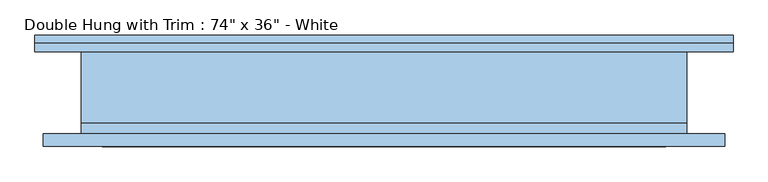
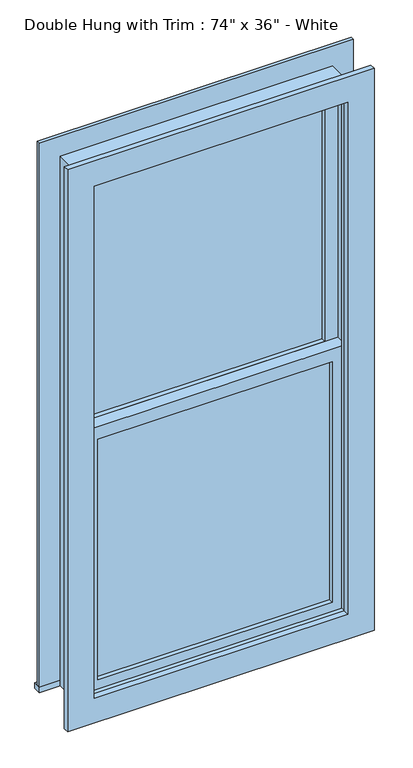
"""IFC4 building model written with IfcOpenShell, lengths in millimetres: window geometry."""

from ifc_helpers import new_model, si_unit, frame, origin, place, context, project, spatial, polyline, outline, extrude, source, transform, mapped, element, save


def window_b8726e58(model_context):
    return source(origin(), model_context, "Body", "SweptSolid", [
        extrude(outline(polyline([(-393.7, -17.4625), (393.7, -17.4625), (393.7, -30.1625), (-393.7, -30.1625), (-393.7, -17.4625)])), frame((0.0, 0.0, 571.5), z_axis=(0.0, 0.0, 1.0), x_axis=(1.0, 0.0, 0.0)), (0.0, 0.0, 1.0), 854.075),
        extrude(outline(polyline([(1470.025, -438.15), (527.05, -438.15), (527.05, 438.15), (1470.025, 438.15), (1470.025, -438.15)]), holes=[polyline([(1425.575, -393.7), (1425.575, 393.7), (571.5, 393.7), (571.5, -393.7), (1425.575, -393.7)])]), frame((0.0, -46.0375, 0.0), z_axis=(0.0, 1.0, 0.0), x_axis=(0.0, 0.0, 1.0)), (0.0, 0.0, 1.0), 44.45),
        extrude(outline(polyline([(-527.05, 87.3125), (527.05, 87.3125), (527.05, 61.9125), (-527.05, 61.9125), (-527.05, 87.3125)])), frame((0.0, 0.0, 508.0), z_axis=(0.0, 0.0, 1.0), x_axis=(1.0, 0.0, 0.0)), (0.0, 0.0, 1.0), 19.05),
        extrude(outline(polyline([(2368.55, -438.15), (2368.55, 438.15), (527.05, 438.15), (527.05, 527.05), (2457.45, 527.05), (2457.45, -527.05), (527.05, -527.05), (527.05, -438.15), (2368.55, -438.15)])), frame((0.0, 61.9125, 0.0), z_axis=(0.0, 1.0, 0.0), x_axis=(0.0, 0.0, 1.0)), (0.0, 0.0, 1.0), 12.7),
        extrude(outline(polyline([(2444.75, 514.35), (2444.75, -514.35), (450.85, -514.35), (450.85, 514.35), (2444.75, 514.35)]), holes=[polyline([(2355.85, 425.45), (539.75, 425.45), (539.75, -425.45), (2355.85, -425.45), (2355.85, 425.45)])]), frame((0.0, -80.9625, 0.0), z_axis=(0.0, 1.0, 0.0), x_axis=(0.0, 0.0, 1.0)), (0.0, 0.0, 1.0), 19.05),
        extrude(outline(polyline([(393.7, 14.2875), (-393.7, 14.2875), (-393.7, 26.9875), (393.7, 26.9875), (393.7, 14.2875)])), frame((0.0, 0.0, 1470.025), z_axis=(0.0, 0.0, 1.0), x_axis=(1.0, 0.0, 0.0)), (0.0, 0.0, 1.0), 854.075),
        extrude(outline(polyline([(2368.55, -438.15), (1425.575, -438.15), (1425.575, 438.15), (2368.55, 438.15), (2368.55, -438.15)]), holes=[polyline([(2324.1, -393.7), (2324.1, 393.7), (1470.025, 393.7), (1470.025, -393.7), (2324.1, -393.7)])]), frame((0.0, -1.5875, 0.0), z_axis=(0.0, 1.0, 0.0), x_axis=(0.0, 0.0, 1.0)), (0.0, 0.0, 1.0), 44.45),
        extrude(outline(polyline([(2387.6, -457.2), (508.0, -457.2), (508.0, 457.2), (2387.6, 457.2), (2387.6, -457.2)]), holes=[polyline([(2355.85, -425.45), (2355.85, 425.45), (539.75, 425.45), (539.75, -425.45), (2355.85, -425.45)])]), frame((0.0, -61.9125, 0.0), z_axis=(0.0, 1.0, 0.0), x_axis=(0.0, 0.0, 1.0)), (0.0, 0.0, 1.0), 15.875),
        extrude(outline(polyline([(2387.6, 457.2), (2387.6, -457.2), (508.0, -457.2), (508.0, 457.2), (2387.6, 457.2)]), holes=[polyline([(2368.55, 438.15), (527.05, 438.15), (527.05, -438.15), (2368.55, -438.15), (2368.55, 438.15)])]), frame((0.0, -46.0375, 0.0), z_axis=(0.0, 1.0, 0.0), x_axis=(0.0, 0.0, 1.0)), (0.0, 0.0, 1.0), 107.95),
    ])


if __name__ == "__main__":
    model = new_model("IFC4")
    model_context = context("Model", 3, world=origin())
    ifc_project = project(units=[si_unit("LENGTHUNIT", "METRE", prefix="MILLI")], contexts=[model_context])
    site = spatial("IfcSite", under=ifc_project)
    building = spatial("IfcBuilding", under=site)
    placement = place(None, origin())
    window_shape = window_b8726e58(model_context)
    element("IfcWindow", 1, ObjectType="Double Hung with Trim : 74\" x 36\" - White", at=placement, inside=building, context=model_context, shape_type="MappedRepresentation", body=[
        mapped(window_shape, transform((0.0, 0.0, 0.0), x_axis=(1.0, 0.0, 0.0), y_axis=(0.0, 1.0, 0.0), z_axis=(0.0, 0.0, 1.0))),
    ])
    save(model, "model.ifc")

# Revit data of these elements
# Type "Double Hung with Trim : 74\" x 36\" - White"
#   Type Mark = "23"
#   COBie.Type.CreatedBy = "doug.wood@us.ibm.com"
#   COBie.Type.CreatedOn = "2016-04-14T02:07:26"
#   COBie.Type.Name = "Windows_Double Hung with Trim_74\" x 36\"_23"
#   COBie.Type.Category = "23-30 20 17 17 14 : Double-Hung Windows"
#   COBie.Type.Description = "Double Hung with Trim_74\" x 36\""
#   COBie.Type.Manufacturer = ""
#   COBie.Type.ModelNumber = ""
#   Construction Type Id = "GSP4R"
#   Assembly Code = "B2020100"
#   Analytic Construction = "1/8 in Pilkington single glazing"
#   COBie.Type.ReplacementCost = 0
#   Visual Light Transmittance = 0.9
#   Solar Heat Gain Coefficient = 0.78
#   Heat Transfer Coefficient (U) = 3.6886 W/(m²·K)
#   Height = 6' - 2"
#   Default Sill Height = 1' - 8"
#   Trim Projection - Ext. = 0' - 0 1/2"
#   Trim Projection - Int. = 0' - 0 3/4"
#   Trim Width - Exterior = 0' - 3 1/2"
#   Trim Width - Interior = 0' - 3 1/2"
#   Width = 3' - 0"
#   Window Inset = 0' - 0 3/4"
#   COBie.Type = no
#   Glass Pane Material = Glass
#   Sash Material = Sash - White
#   Trim Exterior Material = Trim - White
#   Trim Interior Material = Trim - White
#   Wall Closure = (empty or 0)
# Element 1 (IfcWindow, "Double Hung with Trim : 74\" x 36\" - White")
#   Materials on its faces: "Sash - White", "Trim - White", "Glass"
# Materials
#   "Glass": class "Glass", colour RGB 0 128 192, transparency 0.75, Description = "Soda Lime Glass", Cost = 0
#   "Sash - White": class "Wood", colour RGB 255 255 255, transparency 0, Cost = 0
#   "Trim - White": class "Wood", colour RGB 255 255 255, transparency 0, Cost = 0
